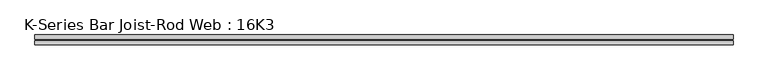
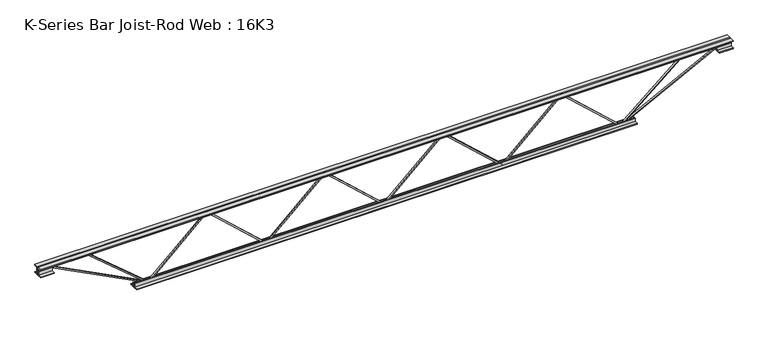
"""IFC4 building model written with IfcOpenShell, lengths in millimetres: beam geometry, K-Series Bar Joist-Rod Web : 16K3."""

from ifc_helpers import new_model, si_unit, frame, origin, place, context, project, spatial, polyline, outline, extrude, source, transform, mapped, element, save


def k_series_bar_joist_rod_web_16k3_52b199ef(model_context):
    return source(origin(), model_context, "Body", "SweptSolid", [
        extrude(outline(polyline([(-192.0875, 0.0), (-201.6125, 0.0), (-201.6125, 5.0202181), (192.0875, 436.8202181), (192.0875, 439.4797819), (-201.6125, 871.2797819), (-201.6125, 876.3), (-192.0875, 876.3), (-192.0875, 874.9702181), (201.6125, 443.1702181), (201.6125, 433.1297819), (-192.0875, 1.3297819), (-192.0875, 0.0)])), frame((0.0, -4.7625, 0.0), z_axis=(0.0, 1.0, 0.0), x_axis=(0.0, 0.0, 1.0)), (0.0, 0.0, 1.0), 9.525),
        extrude(outline(polyline([(-192.0875, -876.3), (-201.6125, -876.3), (-201.6125, -871.2797819), (192.0875, -439.4797819), (192.0875, -436.8202181), (-201.6125, -5.0202181), (-201.6125, 0.0), (-192.0875, 0.0), (-192.0875, -1.3297819), (201.6125, -433.1297819), (201.6125, -443.1702181), (-192.0875, -874.9702181), (-192.0875, -876.3)])), frame((0.0, -4.7625, 0.0), z_axis=(0.0, 1.0, 0.0), x_axis=(0.0, 0.0, 1.0)), (0.0, 0.0, 1.0), 9.525),
        extrude(outline(polyline([(-192.0875, 876.3), (-201.6125, 876.3), (-201.6125, 881.3202181), (192.0875, 1313.1202181), (192.0875, 1315.7797819), (-201.6125, 1747.5797819), (-201.6125, 1752.6), (-192.0875, 1752.6), (-192.0875, 1751.2702181), (201.6125, 1319.4702181), (201.6125, 1309.4297819), (-192.0875, 877.6297819), (-192.0875, 876.3)])), frame((0.0, -4.7625, 0.0), z_axis=(0.0, 1.0, 0.0), x_axis=(0.0, 0.0, 1.0)), (0.0, 0.0, 1.0), 9.525),
        extrude(outline(polyline([(-192.0875, -1752.6), (-201.6125, -1752.6), (-201.6125, -1747.5797819), (192.0875, -1315.7797819), (192.0875, -1313.1202181), (-201.6125, -881.3202181), (-201.6125, -876.3), (-192.0875, -876.3), (-192.0875, -877.6297819), (201.6125, -1309.4297819), (201.6125, -1319.4702181), (-192.0875, -1751.2702181), (-192.0875, -1752.6)])), frame((0.0, -4.7625, 0.0), z_axis=(0.0, 1.0, 0.0), x_axis=(0.0, 0.0, 1.0)), (0.0, 0.0, 1.0), 9.525),
        extrude(outline(polyline([(4.7625, 203.2), (36.5125, 203.2), (36.5125, 196.85), (11.1125, 196.85), (11.1125, 171.45), (4.7625, 171.45), (4.7625, 203.2)])), frame((-2565.4, 0.0, 0.0), z_axis=(1.0, 0.0, 0.0), x_axis=(0.0, 1.0, 0.0)), (0.0, 0.0, 1.0), 5130.8),
        extrude(outline(polyline([(-4.7625, 203.2), (-4.7625, 171.45), (-11.1125, 171.45), (-11.1125, 196.85), (-36.5125, 196.85), (-36.5125, 203.2), (-4.7625, 203.2)])), frame((-2565.4, 0.0, 0.0), z_axis=(1.0, 0.0, 0.0), x_axis=(0.0, 1.0, 0.0)), (0.0, 0.0, 1.0), 5130.8),
        extrude(outline(polyline([(-4.7625, 139.7), (-36.5125, 139.7), (-36.5125, 146.05), (-11.1125, 146.05), (-11.1125, 171.45), (-4.7625, 171.45), (-4.7625, 139.7)])), frame((-2565.4, 0.0, 0.0), z_axis=(1.0, 0.0, 0.0), x_axis=(0.0, 1.0, 0.0)), (0.0, 0.0, 1.0), 101.6),
        extrude(outline(polyline([(36.5125, 139.7), (4.7625, 139.7), (4.7625, 171.45), (11.1125, 171.45), (11.1125, 146.05), (36.5125, 146.05), (36.5125, 139.7)])), frame((-2565.4, 0.0, 0.0), z_axis=(1.0, 0.0, 0.0), x_axis=(0.0, 1.0, 0.0)), (0.0, 0.0, 1.0), 101.6),
        extrude(outline(polyline([(4.7625, 139.7), (4.7625, 171.45), (11.1125, 171.45), (11.1125, 146.05), (36.5125, 146.05), (36.5125, 139.7), (4.7625, 139.7)])), frame((2463.8, 0.0, 0.0), z_axis=(1.0, 0.0, 0.0), x_axis=(0.0, 1.0, 0.0)), (0.0, 0.0, 1.0), 101.6),
        extrude(outline(polyline([(-4.7625, 139.7), (-36.5125, 139.7), (-36.5125, 146.05), (-11.1125, 146.05), (-11.1125, 171.45), (-4.7625, 171.45), (-4.7625, 139.7)])), frame((2463.8, 0.0, 0.0), z_axis=(1.0, 0.0, 0.0), x_axis=(0.0, 1.0, 0.0)), (0.0, 0.0, 1.0), 101.6),
        extrude(outline(polyline([(4.7625, -203.2), (4.7625, -171.45), (11.1125, -171.45), (11.1125, -196.85), (36.5125, -196.85), (36.5125, -203.2), (4.7625, -203.2)])), frame((-1854.2, 0.0, 0.0), z_axis=(1.0, 0.0, 0.0), x_axis=(0.0, 1.0, 0.0)), (0.0, 0.0, 1.0), 3708.4),
        extrude(outline(polyline([(-4.7625, -203.2), (-36.5125, -203.2), (-36.5125, -196.85), (-11.1125, -196.85), (-11.1125, -171.45), (-4.7625, -171.45), (-4.7625, -203.2)])), frame((-1854.2, 0.0, 0.0), z_axis=(1.0, 0.0, 0.0), x_axis=(0.0, 1.0, 0.0)), (0.0, 0.0, 1.0), 3708.4),
        extrude(outline(polyline([(0.0, -9.525), (0.0, 0.0), (800.9059433, 0.0), (800.9059433, -9.525), (0.0, -9.525)])), frame((-2465.9900559, 4.7625, 167.2209266), z_axis=(0.459854247661137, 0.0, 0.8879944092774513), x_axis=(0.8879944092774513, 0.0, -0.459854247661137)), (0.0, 0.0, 1.0), 9.525),
        extrude(outline(polyline([(0.0, -9.525), (0.0, 0.0), (572.381265, 0.0), (572.381265, -9.525), (0.0, -9.525)])), frame((-2193.8144412, 4.7625, 167.8043716), z_axis=(0.6434522276209605, 0.0, 0.7654862707910728), x_axis=(0.7654862707910728, 0.0, -0.6434522276209605)), (0.0, 0.0, 1.0), 9.525),
        extrude(outline(polyline([(0.0, -9.525), (0.0, 0.0), (800.9059433, 0.0), (800.9059433, -9.525), (0.0, -9.525)])), frame((2465.9900559, -4.7625, 167.2209266), z_axis=(-0.4598542476611245, 0.0, 0.8879944092774578), x_axis=(-0.8879944092774578, 0.0, -0.4598542476611245)), (0.0, 0.0, 1.0), 9.525),
        extrude(outline(polyline([(0.0, -9.525), (0.0, 0.0), (572.381265, 0.0), (572.381265, -9.525), (0.0, -9.525)])), frame((2193.8144412, -4.7625, 167.8043716), z_axis=(-0.6434522276209566, 0.0, 0.7654862707910762), x_axis=(-0.7654862707910762, 0.0, -0.6434522276209566)), (0.0, 0.0, 1.0), 9.525),
    ])


if __name__ == "__main__":
    model = new_model("IFC4")
    model_context = context("Model", 3, world=origin())
    ifc_project = project(units=[si_unit("LENGTHUNIT", "METRE", prefix="MILLI")], contexts=[model_context])
    site = spatial("IfcSite", under=ifc_project)
    building = spatial("IfcBuilding", under=site)
    placement = place(None, origin())
    k_series_bar_joist_rod_web_16k3_shape = k_series_bar_joist_rod_web_16k3_52b199ef(model_context)
    element("IfcBeam", 1, ObjectType="K-Series Bar Joist-Rod Web : 16K3", at=placement, inside=building, context=model_context, shape_type="MappedRepresentation", body=[
        mapped(k_series_bar_joist_rod_web_16k3_shape, transform((0.0, 0.0, 0.0), x_axis=(1.0, 0.0, 0.0), y_axis=(0.0, 1.0, 0.0), z_axis=(0.0, 0.0, 1.0))),
    ])
    save(model, "model.ifc")

# Revit data of these elements
# Type "K-Series Bar Joist-Rod Web : 16K3"
#   Assembly Code = "B1010350"
#   Wt = 6.3
#   Web Thickness = 0' - 0 3/8"
#   Start Offset [instance default] = 0' - 0"
#   Start Extension [instance default] = 0' - 0"
#   Seat Length = 0' - 4"
#   Seat Depth = 0' - 2 1/2"
#   PanelArrayLength [instance default] = 18' - 8"
#   Panel [instance default] = 2' - 8"
#   End Offset [instance default] = 0' - 0"
#   End Extension [instance default] = 0' - 0"
#   End Panel = 2' - 8"
#   Cord Leg = 0' - 1 1/4"
#   Chord Thickness = 0' - 0 1/4"
#   Length [instance default] = 24' - 0"
#   Depth = 1' - 4"
#   PanelArrayNum [instance default] = 7
#   Structural Material = none
# Element 1 (IfcBeam, "K-Series Bar Joist-Rod Web : 16K3")
#   PanelArrayLength = 11' - 6"
#   Panel = 2' - 10 1/2"
#   PanelArrayNum = 4
